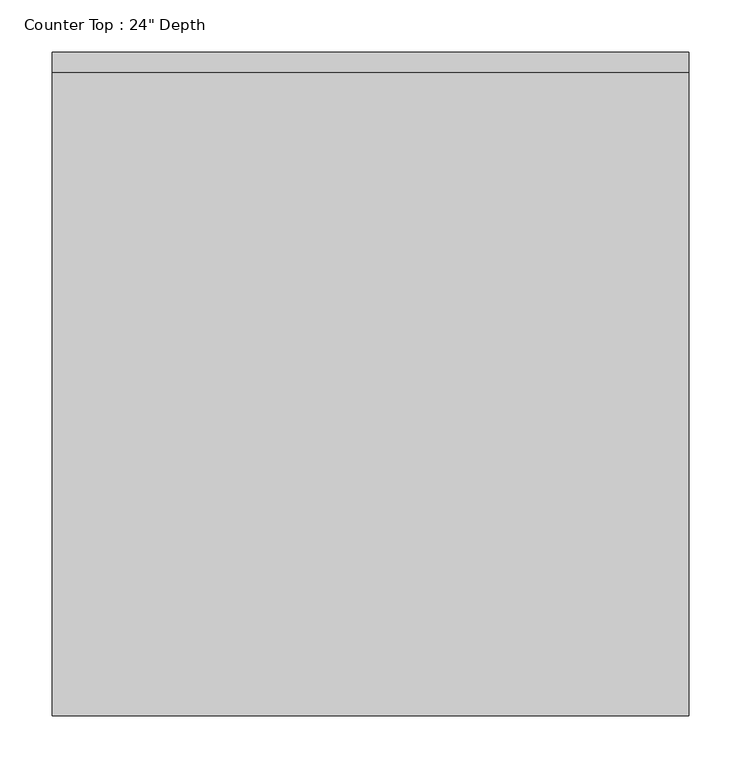
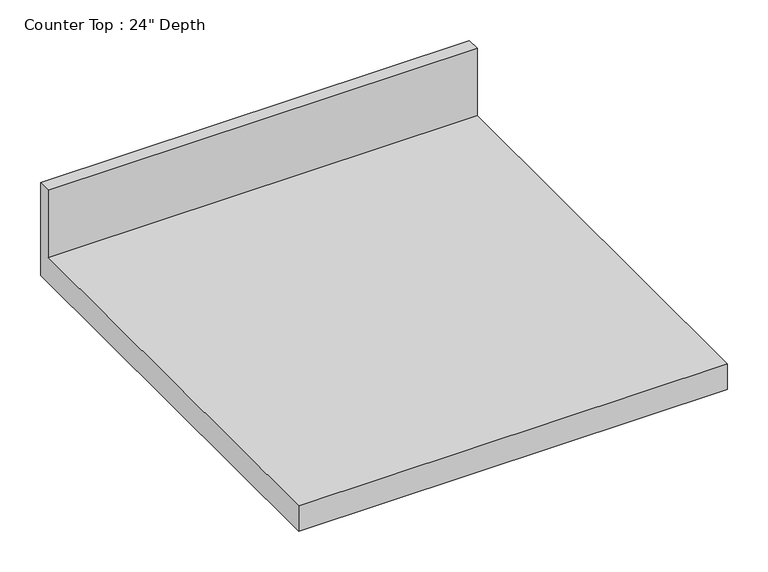
"""IFC4 building model written with IfcOpenShell, lengths in millimetres: furniture geometry."""

from ifc_helpers import new_model, si_unit, frame, origin, place, context, project, spatial, polyline, outline, extrude, source, transform, mapped, element, save


def furniture_86fdc022(model_context):
    return source(origin(), model_context, "Body", "SweptSolid", [
        extrude(outline(polyline([(0.0, 1016.0), (0.0, 876.3), (-635.0, 876.3), (-635.0, 914.4), (-19.05, 914.4), (-19.05, 1016.0), (0.0, 1016.0)])), frame((-1200.4622951, 0.0, 0.0), z_axis=(1.0, 0.0, 0.0), x_axis=(0.0, 1.0, 0.0)), (0.0, 0.0, 1.0), 609.6),
    ])


if __name__ == "__main__":
    model = new_model("IFC4")
    model_context = context("Model", 3, world=origin())
    ifc_project = project(units=[si_unit("LENGTHUNIT", "METRE", prefix="MILLI")], contexts=[model_context])
    site = spatial("IfcSite", under=ifc_project)
    building = spatial("IfcBuilding", under=site)
    placement = place(None, origin())
    furniture_shape = furniture_86fdc022(model_context)
    element("IfcFurniture", 1, ObjectType="Counter Top : 24\" Depth", at=placement, inside=building, context=model_context, shape_type="MappedRepresentation", body=[
        mapped(furniture_shape, transform((0.0, 0.0, 0.0), x_axis=(1.0, 0.0, 0.0), y_axis=(0.0, 1.0, 0.0), z_axis=(0.0, 0.0, 1.0))),
    ])
    save(model, "model.ifc")

# Revit data of these elements
# Type "Counter Top : 24\" Depth"
#   Assembly Code = "C1030400"
#   Counter Thickness = 0' - 1 1/2"
#   Depth = 2' - 1"
#   Height = 3' - 0"
#   Length [instance default] = 8' - 0"
#   Counter Top Material = Laminate, Blue, Matte
#   Default Elevation = 0
# Element 1 (IfcFurniture, "Counter Top : 24\" Depth")
#   Length = 2' - 0"
#   Materials on its faces: "Laminate, Blue, Matte"
# Materials
#   "Laminate, Blue, Matte": class "Plastic", colour RGB 85 101 155, transparency 0, Description = "Plastic Laminate - Blue, Matte", Cost = 0
